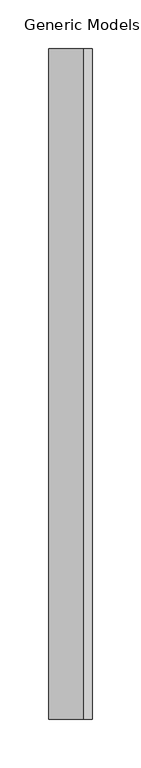
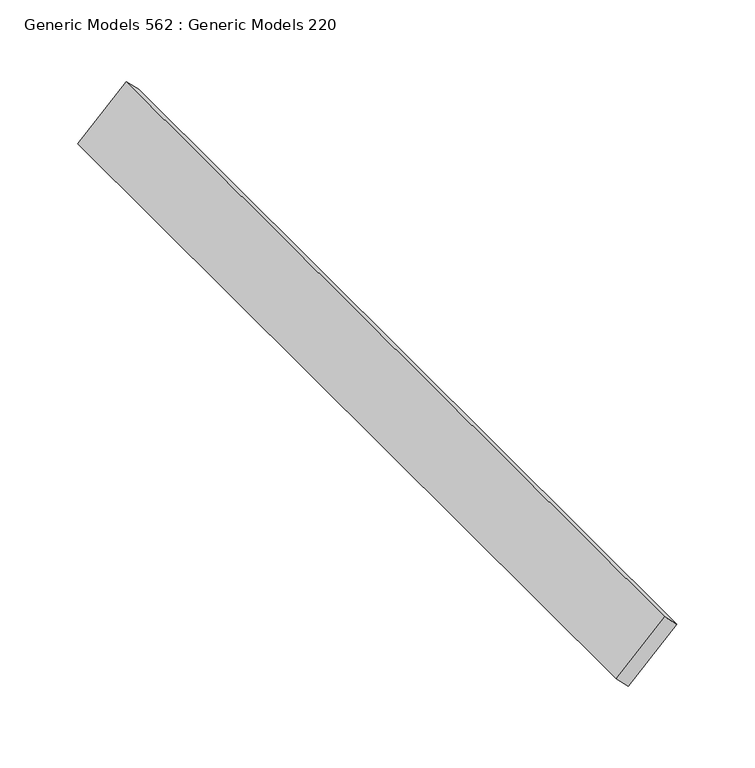
"""IFC4 building model written with IfcOpenShell, lengths in millimetres: proxy geometry, Generic Models 562 : Generic Models 220."""

from ifc_helpers import new_model, si_unit, frame, origin, place, context, project, spatial, polyline, outline, extrude, source, transform, mapped, element, save


def generic_models_562_generic_models_220_78eec420(model_context):
    return source(origin(), model_context, "Body", "SweptSolid", [
        extrude(outline(polyline([(0.0, -12.7000001), (0.0, 0.0), (690.8142348, 0.0), (690.8142348, -12.7000001), (0.0, -12.7000001)])), frame((7841.3059863, 4539.4872686, 124303.1399101), z_axis=(0.7071067811868034, 0.0, 0.7071067811862918), x_axis=(0.0, -1.0, 0.0)), (0.0, 0.0, 1.0), 50.8),
    ])


if __name__ == "__main__":
    model = new_model("IFC4")
    model_context = context("Model", 3, world=origin())
    ifc_project = project(units=[si_unit("LENGTHUNIT", "METRE", prefix="MILLI")], contexts=[model_context])
    site = spatial("IfcSite", under=ifc_project)
    building = spatial("IfcBuilding", under=site)
    placement = place(None, origin())
    generic_models_562_generic_models_220_shape = generic_models_562_generic_models_220_78eec420(model_context)
    element("IfcBuildingElementProxy", 1, Name="Generic Models 562 : Generic Models 220", ObjectType="Generic Models 562 : Generic Models 220", at=placement, inside=building, context=model_context, shape_type="MappedRepresentation", body=[
        mapped(generic_models_562_generic_models_220_shape, transform((0.0, 0.0, 0.0), x_axis=(1.0, 0.0, 0.0), y_axis=(0.0, 1.0, 0.0), z_axis=(0.0, 0.0, 1.0))),
    ])
    save(model, "model.ifc")

# Revit data of these elements
# Element 1 (IfcBuildingElementProxy, "Generic Models 562 : Generic Models 220")
#   Materials on its faces: "_WOOD TONE ALUMINUM EXTRUSION SLAT BY KNOTWOOD"
# Materials
#   "_WOOD TONE ALUMINUM EXTRUSION SLAT BY KNOTWOOD": class "Generic", colour RGB 177 130 114, transparency 0, Cost = 0
